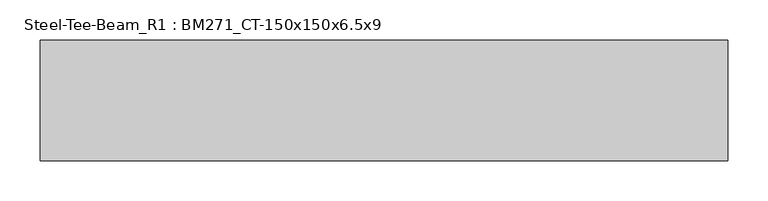
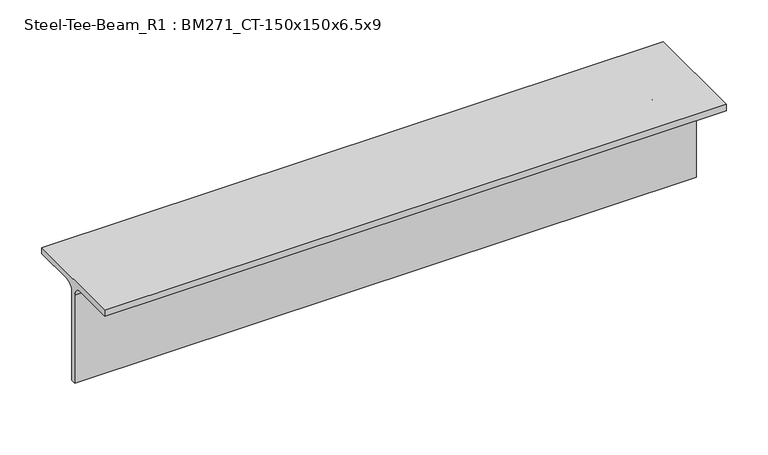
"""IFC4 building model written with IfcOpenShell, lengths in millimetres: member geometry, Steel-Tee-Beam_R1 : BM271_CT-150x150x6.5x9."""

from ifc_helpers import new_model, si_unit, point, frame, frame_2d, origin, place, context, project, spatial, polyline, circle_curve, trimmed, segment, composite_curve, outline, extrude, source, transform, mapped, element, save


def steel_tee_beam_r1_bm271_ct_150x150x6_5x9_0e9b9814(model_context):
    return source(origin(), model_context, "Body", "SweptSolid", [
        extrude(outline(composite_curve([segment(polyline([(75.0, 75.0), (75.0, 66.0), (16.25, 66.0)]), True, "CONTINUOUS"), segment(trimmed(circle_curve(frame_2d((16.25, 53.0)), 13.0), [point((16.25, 66.0))], [point((3.25, 53.0))], True, "CARTESIAN"), True, "CONTINUOUS"), segment(polyline([(3.25, 53.0), (3.25, -75.0), (-3.25, -75.0), (-3.25, 53.0)]), True, "CONTINUOUS"), segment(trimmed(circle_curve(frame_2d((-16.25, 53.0)), 13.0), [point((-3.25, 53.0))], [point((-16.25, 66.0))], True, "CARTESIAN"), True, "CONTINUOUS"), segment(polyline([(-16.25, 66.0), (-75.0, 66.0), (-75.0, 75.0), (75.0, 75.0)]), True, "CONTINUOUS")], self_intersect=False)), frame((-500.0, 0.0, 0.0), z_axis=(1.0, 0.0, 0.0), x_axis=(0.0, 1.0, 0.0)), (0.0, 0.0, 1.0), 856.1687518),
    ])


if __name__ == "__main__":
    model = new_model("IFC4")
    model_context = context("Model", 3, world=origin())
    ifc_project = project(units=[si_unit("LENGTHUNIT", "METRE", prefix="MILLI")], contexts=[model_context])
    site = spatial("IfcSite", under=ifc_project)
    building = spatial("IfcBuilding", under=site)
    placement = place(None, origin())
    steel_tee_beam_r1_bm271_ct_150x150x6_5x9_shape = steel_tee_beam_r1_bm271_ct_150x150x6_5x9_0e9b9814(model_context)
    element("IfcMember", 1, ObjectType="Steel-Tee-Beam_R1 : BM271_CT-150x150x6.5x9", at=placement, inside=building, context=model_context, shape_type="MappedRepresentation", body=[
        mapped(steel_tee_beam_r1_bm271_ct_150x150x6_5x9_shape, transform((0.0, 0.0, 0.0), x_axis=(1.0, 0.0, 0.0), y_axis=(0.0, 1.0, 0.0), z_axis=(0.0, 0.0, 1.0))),
    ])
    save(model, "model.ifc")

# Revit data of these elements
# Type "Steel-Tee-Beam_R1 : BM271_CT-150x150x6.5x9"
#   Keynote = "CT-150x150x6.5x9"
#   Surface Area = 0.588841 m²/m
#   Section Area = 23.3904 cm²
#   Mass per Unit Length = 18.3614 kg/m
#   Length [instance default] = 1.5240 m
#   bf = 0.1500 m
#   d = 0.1500 m
#   k = 0.0220 m
#   r = 0.0130 m
#   tf = 0.0090 m
#   tw = 0.0065 m
#   hec_material4 [instance default] = none
#   hec_material3 [instance default] = none
#   hec_material2 [instance default] = none
#   hec_material1 [instance default] = none
#   Structural Material [instance default] = Steel, 45-345
#   Assembly Code = ""
# Element 1 (IfcMember, "Steel-Tee-Beam_R1 : BM271_CT-150x150x6.5x9")
#   Structural Material = none
# Materials
#   "Steel, 45-345": class "Metal", colour RGB 189 187 185, transparency 0, Description = "Steel 345 MPa", Cost = 0
